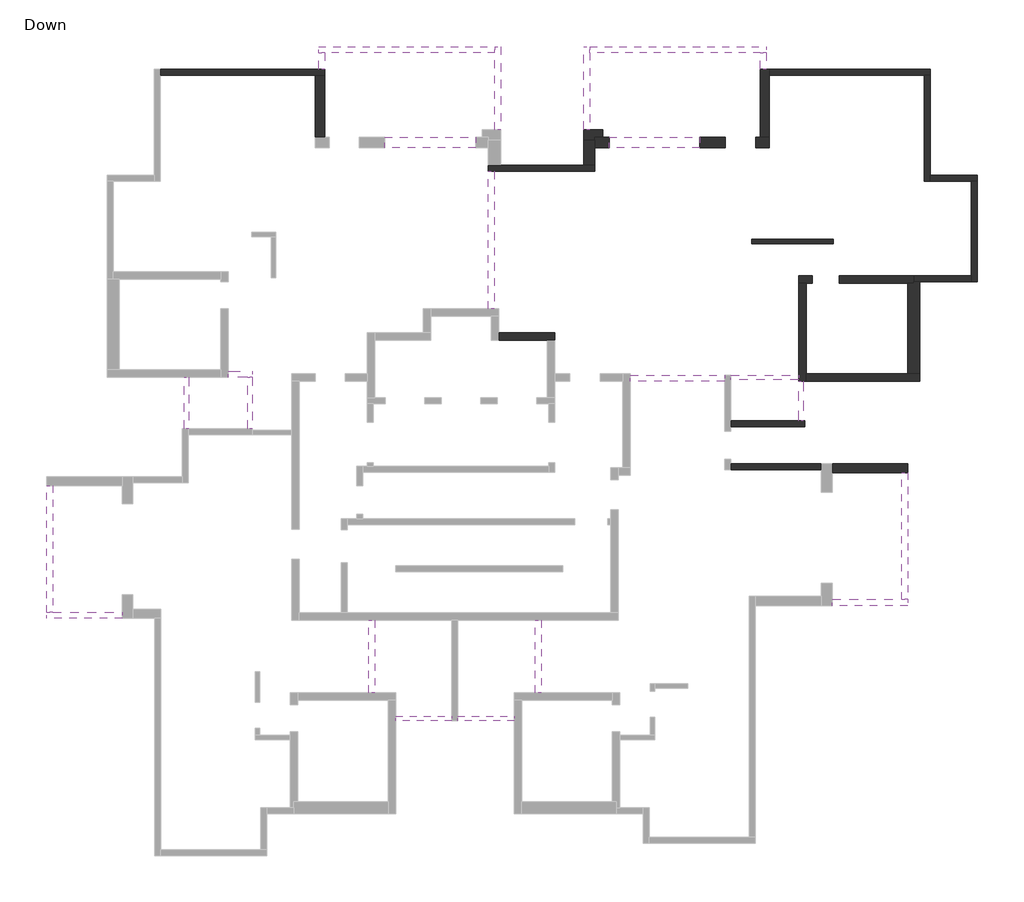
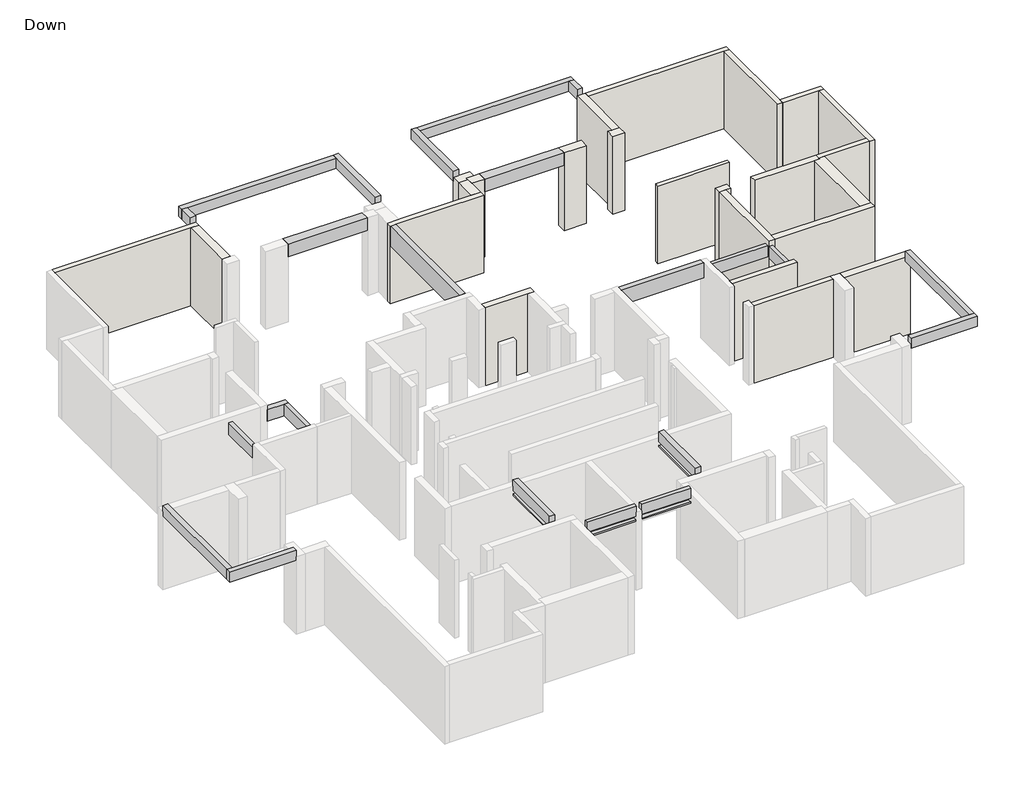
# One storey, part 3 of 3: 24 walls, 23 beams.
# Revit data of these elements (continued)
# Element 38 (IfcWall, "25") (continued)
#   Top Offset = 0 cm
#   Base Offset = 0 cm
#   wall height = 310 cm
#   SOFiSTiK_AMG_Scheduled = yes
#   SOFiSTiK_AMG_Adjusted = yes
#   Phase Created = New Construction
#   Base Constraint = Down
#   Top Constraint = Typical Floor
#   Materials on its faces: "Concrete"
# Element 39 (IfcWall, "30")
#   Comments = ""
#   Mark = "W43"
#   SOFiSTiK_EdgeZones = "W43"
#   SOFiSTiK_AMG_Comments = ""
#   Top Offset = 0 cm
#   Base Offset = 0 cm
#   wall height = 310 cm
#   SOFiSTiK_AMG_Scheduled = yes
#   SOFiSTiK_AMG_Adjusted = yes
#   Phase Created = New Construction
#   Base Constraint = Down
#   Top Constraint = Typical Floor
#   Materials on its faces: "Concrete"
# Element 40 (IfcWall, "30")
#   Comments = ""
#   Mark = "W47"
#   SOFiSTiK_EdgeZones = "W47"
#   SOFiSTiK_AMG_Comments = ""
#   Top Offset = 0 cm
#   Base Offset = 0 cm
#   wall height = 310 cm
#   SOFiSTiK_AMG_Scheduled = yes
#   SOFiSTiK_AMG_Adjusted = yes
#   Phase Created = New Construction
#   Base Constraint = Down
#   Top Constraint = Typical Floor
#   Materials on its faces: "Concrete"
# Element 41 (IfcWall, "30")
#   Comments = ""
#   Mark = "W48"
#   SOFiSTiK_EdgeZones = "W48"
#   SOFiSTiK_AMG_Comments = ""
#   Top Offset = 0 cm
#   Base Offset = 0 cm
#   wall height = 310 cm
#   SOFiSTiK_AMG_Scheduled = yes
#   SOFiSTiK_AMG_Adjusted = yes
#   Phase Created = New Construction
#   Base Constraint = Down
#   Top Constraint = Typical Floor
#   Materials on its faces: "Concrete"
# Element 42 (IfcWall, "35")
#   Comments = ""
#   Mark = "W55"
#   SOFiSTiK_EdgeZones = "W55"
#   SOFiSTiK_AMG_Comments = ""
#   Top Offset = 0 cm
#   Base Offset = 0 cm
#   wall height = 310 cm
#   SOFiSTiK_AMG_Scheduled = yes
#   SOFiSTiK_AMG_Adjusted = yes
#   Phase Created = New Construction
#   Base Constraint = Down
#   Top Constraint = Typical Floor
#   Materials on its faces: "Concrete"
# Element 43 (IfcWall, "35")
#   Comments = ""
#   Mark = "W56"
#   SOFiSTiK_EdgeZones = "W56"
#   SOFiSTiK_AMG_Comments = ""
#   Top Offset = 0 cm
#   Base Offset = 0 cm
#   wall height = 310 cm
#   SOFiSTiK_AMG_Scheduled = yes
#   SOFiSTiK_AMG_Adjusted = yes
#   Phase Created = New Construction
#   Base Constraint = Down
#   Top Constraint = Typical Floor
#   Materials on its faces: "Concrete"
# Element 44 (IfcWall, "35")
#   Comments = ""
#   Mark = "W57"
#   SOFiSTiK_EdgeZones = "W57"
#   SOFiSTiK_AMG_Comments = ""
#   Top Offset = 0 cm
#   Base Offset = 0 cm
#   wall height = 310 cm
#   SOFiSTiK_AMG_Scheduled = yes
#   SOFiSTiK_AMG_Adjusted = yes
#   Phase Created = New Construction
#   Base Constraint = Down
#   Top Constraint = Typical Floor
#   Materials on its faces: "Concrete"
# Element 45 (IfcWall, "35")
#   Comments = ""
#   Mark = "W58"
#   SOFiSTiK_EdgeZones = "W58"
#   SOFiSTiK_AMG_Comments = ""
#   Top Offset = 0 cm
#   Base Offset = 0 cm
#   wall height = 310 cm
#   SOFiSTiK_AMG_Scheduled = yes
#   SOFiSTiK_AMG_Adjusted = yes
#   Phase Created = New Construction
#   Base Constraint = Down
#   Top Constraint = Typical Floor
#   Materials on its faces: "Concrete"
# Element 46 (IfcWall, "35")
#   Comments = ""
#   Mark = "W61"
#   SOFiSTiK_EdgeZones = "W61"
#   SOFiSTiK_AMG_Comments = ""
#   Top Offset = 0 cm
#   Base Offset = 0 cm
#   wall height = 310 cm
#   SOFiSTiK_AMG_Scheduled = yes
#   SOFiSTiK_AMG_Adjusted = yes
#   Phase Created = New Construction
#   Base Constraint = Down
#   Top Constraint = Typical Floor
#   Materials on its faces: "Concrete"
# Element 47 (IfcWall, "40")
#   Comments = ""
#   Mark = "W99"
#   SOFiSTiK_EdgeZones = "W103"
#   SOFiSTiK_AMG_Comments = ""
#   Top Offset = 0 cm
#   Base Offset = 0 cm
#   wall height = 310 cm
#   SOFiSTiK_AMG_Scheduled = yes
#   SOFiSTiK_AMG_Adjusted = yes
#   Phase Created = New Construction
#   Base Constraint = Down
#   Top Constraint = Typical Floor
#   Materials on its faces: "Concrete"
# Materials
#   "Concrete": class "Concrete", colour RGB 192 192 192, transparency 0, Keynote = "01000", Description = "Cast-in-place concrete", Cost = 0
